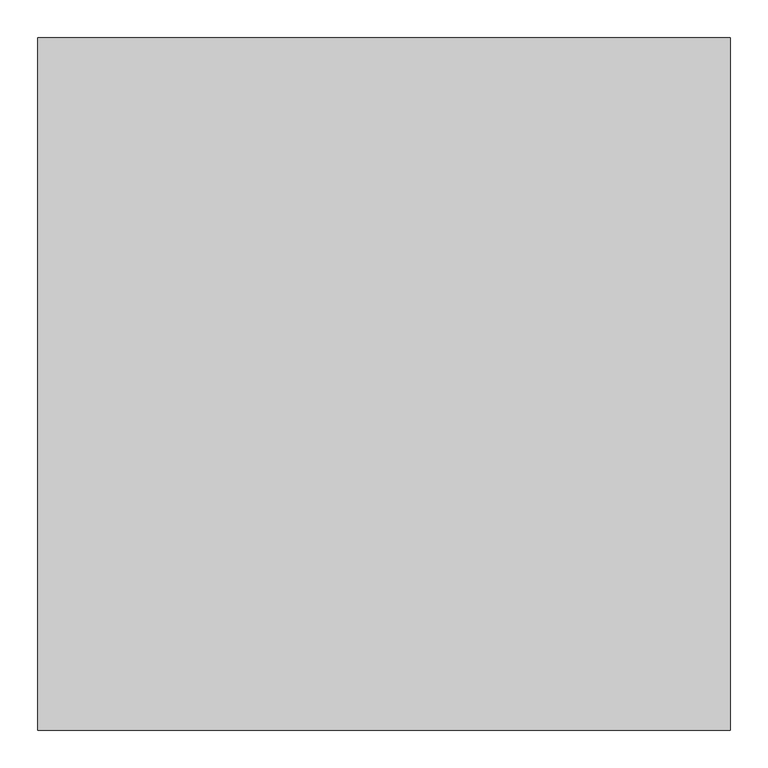
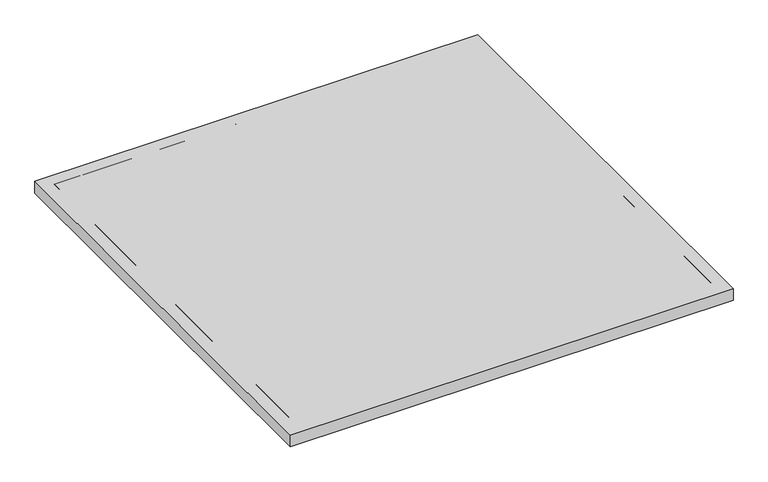
"""IFC4 building model written with IfcOpenShell, lengths in millimetres: proxy geometry, A6046 - Artwork, Decorative, With Frame : A6046 - Artwork, Decorative, With Frame."""

import ifcopenshell
import ifcopenshell.guid

model = None  # the IFC model being written
_history = None  # IfcOwnerHistory: only IFC2X3 demands one
_inside = {}  # id of a spatial element -> (the spatial element, [elements in it])
_under = {}  # id of a project, library or spatial element -> (it, [spatial elements below it])
_declared = {}  # id of a project -> (the project, [libraries it declares])
_typed = {}  # id of a type object -> (the type object, [elements of that type])
_made_of = {}  # id of a material, layer set ... -> (it, [elements and type objects made of it])


def new_model(schema):
    """Start an empty IFC model of exactly this schema.

    Asked for "IFC4X3", IfcOpenShell would pick the latest addendum, in which some entities
    have other attributes; the version numbers below select the first issue.
    IFC2X3 requires an IfcOwnerHistory on every rooted entity: one is made here for all.
    """
    global model, _history
    if schema == "IFC4X3":
        model = ifcopenshell.file(schema_version=(4, 3, 0, 0))
    else:
        model = ifcopenshell.file(schema=schema)
    _inside.clear()
    _under.clear()
    _declared.clear()
    _typed.clear()
    _made_of.clear()
    _history = None
    if model.schema == "IFC2X3":
        org = make("IfcOrganization", Name="unknown")
        user = make(
            "IfcPersonAndOrganization",
            ThePerson=make("IfcPerson", FamilyName="unknown"),
            TheOrganization=org,
        )
        app = make(
            "IfcApplication",
            ApplicationDeveloper=org,
            Version="unknown",
            ApplicationFullName="unknown",
            ApplicationIdentifier="unknown",
        )
        _history = make(
            "IfcOwnerHistory",
            OwningUser=user,
            OwningApplication=app,
            ChangeAction="ADDED",
            CreationDate=0,
        )
    return model


def make(cls, **values):
    """One entity of the class cls with the attributes given. An attribute that is None is left unset."""
    return model.create_entity(
        cls, **{name: value for name, value in values.items() if value is not None}
    )


def rooted(cls, **values):
    """An entity with a GlobalId (a new one), such as an element, a storey or a relation."""
    return make(cls, GlobalId=ifcopenshell.guid.new(), OwnerHistory=_history, **values)


def si_unit(unit_type, name, prefix=None):
    """IfcSIUnit, for example si_unit("LENGTHUNIT", "METRE", prefix="MILLI")."""
    return make("IfcSIUnit", UnitType=unit_type, Prefix=prefix, Name=name)


def assignment(units):
    """IfcUnitAssignment: the units of a project."""
    return None if units is None else make("IfcUnitAssignment", Units=units)


def point(xyz):
    """IfcCartesianPoint."""
    return None if xyz is None else make("IfcCartesianPoint", Coordinates=xyz)


def direction(xyz):
    """IfcDirection."""
    return None if xyz is None else make("IfcDirection", DirectionRatios=xyz)


def frame(location, z_axis=None, x_axis=None):
    """IfcAxis2Placement3D, a coordinate frame: its origin and axes. An axis left out is left unset."""
    return make(
        "IfcAxis2Placement3D",
        Location=point(location),
        Axis=direction(z_axis),
        RefDirection=direction(x_axis),
    )


def origin():
    """The frame at (0, 0, 0) with its axes left unset."""
    return frame((0.0, 0.0, 0.0))


def origin_with_axes():
    """The frame at (0, 0, 0) with the z axis (0, 0, 1) and the x axis (1, 0, 0) written out."""
    return frame((0.0, 0.0, 0.0), z_axis=(0.0, 0.0, 1.0), x_axis=(1.0, 0.0, 0.0))


def place(relative_to, where):
    """IfcLocalPlacement: puts the frame where relative to a parent placement (None: the world)."""
    return make(
        "IfcLocalPlacement", PlacementRelTo=relative_to, RelativePlacement=where
    )


def context(
    kind, dimensions, precision=None, world=None, true_north=None, identifier=None
):
    """IfcGeometricRepresentationContext, for example the 3D "Model" context."""
    return make(
        "IfcGeometricRepresentationContext",
        ContextIdentifier=identifier,
        ContextType=kind,
        CoordinateSpaceDimension=dimensions,
        Precision=precision,
        WorldCoordinateSystem=world,
        TrueNorth=true_north,
    )


def project(units=None, contexts=None):
    """IfcProject with its units and contexts."""
    return rooted(
        "IfcProject",
        Name="project",
        RepresentationContexts=contexts,
        UnitsInContext=assignment(units),
    )


def spatial(cls, under=None, at=None, **own):
    """A site, building, storey or space (cls), placed at a placement, below another one or the project."""
    s = rooted(cls, ObjectPlacement=at, **own)
    if under is not None:
        _under.setdefault(under.id(), (under, []))[1].append(s)
    return s


def polyline(points):
    """IfcPolyline through the points."""
    return make("IfcPolyline", Points=[point(p) for p in points])


def outline(outer, holes=None, kind="AREA"):
    """IfcArbitraryClosedProfileDef: a profile drawn as a closed curve; with holes, ...WithVoids."""
    if holes is None:
        return make("IfcArbitraryClosedProfileDef", ProfileType=kind, OuterCurve=outer)
    return make(
        "IfcArbitraryProfileDefWithVoids",
        ProfileType=kind,
        OuterCurve=outer,
        InnerCurves=holes,
    )


def extrude(swept, where, along, depth):
    """IfcExtrudedAreaSolid: the profile swept, set in the frame where, extruded along a direction by depth."""
    return make(
        "IfcExtrudedAreaSolid",
        SweptArea=swept,
        Position=where,
        ExtrudedDirection=direction(along),
        Depth=depth,
    )


def faces_of(points, faces, orient=None, outer=None):
    """IfcFace entities. A face is a list of loops; a loop is a list of indices into points, from 0.

    orient and outer hold one flag for each loop. By default every Orientation is true, the
    first loop of a face is its IfcFaceOuterBound and the others are IfcFaceBound.
    """
    made = []
    for i, loops in enumerate(faces):
        bounds = []
        for j, loop in enumerate(loops):
            is_outer = j == 0 if outer is None else outer[i][j]
            bounds.append(
                make(
                    "IfcFaceOuterBound" if is_outer else "IfcFaceBound",
                    Bound=make("IfcPolyLoop", Polygon=[points[k] for k in loop]),
                    Orientation=True if orient is None else orient[i][j],
                )
            )
        made.append(make("IfcFace", Bounds=bounds))
    return made


def faceted_brep(points, faces, orient=None, outer=None, voids=None):
    """IfcFacetedBrep: a solid bounded by flat faces; with voids (closed shells), ...WithVoids."""
    shared = [point(p) for p in points]
    hull = make("IfcClosedShell", CfsFaces=faces_of(shared, faces, orient, outer))
    if voids is None:
        return make("IfcFacetedBrep", Outer=hull)
    return make(
        "IfcFacetedBrepWithVoids",
        Outer=hull,
        Voids=[
            make(cls, CfsFaces=faces_of(shared, fs, o, b)) for cls, fs, o, b in voids
        ],
    )


def shape(context_of_items, identifier, shape_type, items):
    """IfcShapeRepresentation: the items that make up one representation, for example the "Body"."""
    return make(
        "IfcShapeRepresentation",
        ContextOfItems=context_of_items,
        RepresentationIdentifier=identifier,
        RepresentationType=shape_type,
        Items=items,
    )


def source(mapping_origin, context_of_items, identifier, shape_type, items):
    """IfcRepresentationMap: a shape defined once, which mapped items show again and again."""
    return make(
        "IfcRepresentationMap",
        MappingOrigin=mapping_origin,
        MappedRepresentation=shape(context_of_items, identifier, shape_type, items),
    )


def transform(
    local_origin,
    x_axis=None,
    y_axis=None,
    z_axis=None,
    scale=None,
    scale2=None,
    scale3=None,
    uniform=True,
):
    """IfcCartesianTransformationOperator3D, or its non-uniform kind. x_axis, y_axis, z_axis: its Axis1, 2, 3."""
    if uniform:
        return make(
            "IfcCartesianTransformationOperator3D",
            Axis1=direction(x_axis),
            Axis2=direction(y_axis),
            LocalOrigin=point(local_origin),
            Scale=scale,
            Axis3=direction(z_axis),
        )
    return make(
        "IfcCartesianTransformationOperator3DnonUniform",
        Axis1=direction(x_axis),
        Axis2=direction(y_axis),
        LocalOrigin=point(local_origin),
        Scale=scale,
        Axis3=direction(z_axis),
        Scale2=scale2,
        Scale3=scale3,
    )


def mapped(mapping_source, mapping_target):
    """IfcMappedItem: shows the shape of a source again, moved by a transform."""
    return make(
        "IfcMappedItem", MappingSource=mapping_source, MappingTarget=mapping_target
    )


def made_of(thing, what):
    """Note that an element or type object is made of a material, layer set ...; save() writes the relation."""
    if what is not None:
        _made_of.setdefault(what.id(), (what, []))[1].append(thing)
    return thing


def element(
    cls,
    number,
    at=None,
    inside=None,
    cuts=None,
    type_object=None,
    material=None,
    context=None,
    identifier="Body",
    shape_type=None,
    held_by="IfcProductDefinitionShape",
    body=None,
    shapes=None,
    **own,
):
    """One element of the class cls, such as IfcWall. Its Tag is "e" and its number.

    at: its placement. inside: the storey or other place that contains it. cuts: it is an
    opening in that element (IfcRelVoidsElement). A single representation is given by context,
    identifier, shape_type and body (its items); several are given by shapes. held_by: the class
    of the entity that holds the representations. save() writes the other relations.
    """
    e = rooted(cls, Tag="e%d" % number, ObjectPlacement=at, **own)
    if body is not None:
        shapes = [shape(context, identifier, shape_type, body)]
    if shapes is not None:
        e.Representation = make(held_by, Representations=shapes)
    if inside is not None:
        _inside.setdefault(inside.id(), (inside, []))[1].append(e)
    if cuts is not None:
        rooted(
            "IfcRelVoidsElement", RelatingBuildingElement=cuts, RelatedOpeningElement=e
        )
    if type_object is not None:
        _typed.setdefault(type_object.id(), (type_object, []))[1].append(e)
    return made_of(e, material)


def aggregate(whole, parts):
    """IfcRelAggregates: a whole, such as a stair, and the parts it consists of."""
    return rooted("IfcRelAggregates", RelatingObject=whole, RelatedObjects=parts)


def save(model, path):
    """Write the relations noted so far, then the file.

    IfcRelAggregates (storeys below a building ...), IfcRelContainedInSpatialStructure (elements
    in a storey), IfcRelDefinesByType, IfcRelAssociatesMaterial and IfcRelDeclares: one each for
    every whole, place, type object, material and project.
    """
    for whole, parts in _under.values():
        aggregate(whole, parts)
    for where, things in _inside.values():
        rooted(
            "IfcRelContainedInSpatialStructure",
            RelatedElements=things,
            RelatingStructure=where,
        )
    for kind, things in _typed.values():
        rooted("IfcRelDefinesByType", RelatedObjects=things, RelatingType=kind)
    for what, things in _made_of.values():
        rooted("IfcRelAssociatesMaterial", RelatedObjects=things, RelatingMaterial=what)
    for by, libraries in _declared.values():
        rooted("IfcRelDeclares", RelatingContext=by, RelatedDefinitions=libraries)
    model.write(path)


def specialty_equipment_89782f33(model_context):
    return source(origin(), model_context, "Body", "SolidModel", [
        extrude(outline(polyline([(457.2, 914.4), (457.2, 0.0), (-457.2, 0.0), (-457.2, 914.4), (457.2, 914.4)])), origin_with_axes(), (0.0, 0.0, 1.0), 25.4),
        extrude(outline(polyline([(431.8, 889.0), (431.8, 25.4), (-431.8, 25.4), (-431.8, 889.0), (431.8, 889.0)])), frame((0.0, 0.0, 12.7), z_axis=(0.0, 0.0, 1.0), x_axis=(1.0, 0.0, 0.0)), (0.0, 0.0, 1.0), 12.7),
        faceted_brep([(457.2, 914.4, 25.4), (457.2, 914.4, 0.0), (-457.2, 914.4, 0.0), (-457.2, 914.4, 25.4), (457.2, 0.0, 25.4), (-457.2, 0.0, 25.4), (-457.2, 0.0, 0.0), (457.2, 0.0, 0.0), (431.8, 889.0, 25.4), (431.8, 25.4, 25.4), (-431.8, 25.4, 25.4), (-431.8, 889.0, 25.4), (-431.8, 889.0, 12.7), (431.8, 889.0, 12.7), (431.8, 25.4, 12.7), (-431.8, 25.4, 12.7)], [[[0, 1, 2, 3]], [[4, 5, 6, 7]], [[3, 5, 4, 0], [8, 9, 10, 11]], [[2, 6, 5, 3]], [[1, 7, 6, 2]], [[0, 4, 7, 1]], [[8, 11, 12, 13]], [[10, 9, 14, 15]], [[11, 10, 15, 12]], [[12, 15, 14, 13]], [[13, 14, 9, 8]]]),
    ])


if __name__ == "__main__":
    model = new_model("IFC4")
    model_context = context("Model", 3, world=origin())
    ifc_project = project(units=[si_unit("LENGTHUNIT", "METRE", prefix="MILLI")], contexts=[model_context])
    site = spatial("IfcSite", under=ifc_project)
    building = spatial("IfcBuilding", under=site)
    placement = place(None, origin())
    specialty_equipment_shape = specialty_equipment_89782f33(model_context)
    element("IfcBuildingElementProxy", 1, Name="A6046 - Artwork, Decorative, With Frame : A6046 - Artwork, Decorative, With Frame", ObjectType="A6046 - Artwork, Decorative, With Frame : A6046 - Artwork, Decorative, With Frame", at=placement, inside=building, context=model_context, shape_type="MappedRepresentation", body=[
        mapped(specialty_equipment_shape, transform((0.0, 0.0, 0.0), x_axis=(1.0, 0.0, 0.0), y_axis=(0.0, 1.0, 0.0), z_axis=(0.0, 0.0, 1.0))),
    ])
    save(model, "model.ifc")

# Revit data of these elements
# Type "A6046 - Artwork, Decorative, With Frame : A6046 - Artwork, Decorative, With Frame"
#   Watts2 = "0"
#   Watts1 = "0"
#   Unit_Issue = "EA"
#   UTIL_6_Misc = "-"
#   UTIL_5_NonMedGas = "-"
#   UTIL_4_MiscGas = "-"
#   UTIL_3_MedGas = "-"
#   UTIL_2_Elec = "-"
#   UTIL_1_WaterDrain = "-"
#   Nomenclature = "Artwork, Decorative, With Frame"
#   NSN = "6230"
#   Location [instance default] = ""
#   JSN = "A6046"
#   Fund_Source_VA = "-"
#   Fund_Source_Navy = "-"
#   Fund_Source_Army = "-"
#   Fund_Source_AF = "-"
#   ELEC_Volts2 = "0"
#   ELEC_Volts1 = "0"
#   ELEC_Phase2 = "0"
#   ELEC_Phase1 = "0"
#   ELEC_HertzSwitch = "0"
#   ELEC_HertzDependent = "0"
#   ELEC_Hertz = "0"
#   ELEC_Amps2 = "0"
#   ELEC_Amps1 = "0"
#   DetailDescription = "This JSN is to be used for determining and defining location of decorative artwork."
#   CAT_VA = "C"
#   CAT_Navy = "C"
#   CAT_IHS = "-"
#   CAT_Army = "C"
#   CAT_AF = "C"
#   BTUperhour = "0"
#   Weight_IP = 0
#   Default Elevation = 7' - 0"
#   DIM_Width_IP = 0' - 0"
#   DIM_Height_IP = 0' - 0"
#   DIM_Depth_IP = 0' - 0"
#   CustomLength [instance default] = 3' - 0"
#   CustomHeight [instance default] = 3' - 0"
# Element 1 (IfcBuildingElementProxy, "A6046 - Artwork, Decorative, With Frame : A6046 - Artwork, Decorative, With Frame")
#   Location = "BRII2"
#   Materials on its faces: "Frame - Wood", "EquipSpace", "Picture"
# Materials
#   "Frame - Wood": class "Miscellaneous", colour RGB 66 39 32, transparency 0
#   "EquipSpace": class "Unassigned", colour RGB 221 217 195, transparency 0.5
#   "Picture": class "Miscellaneous", colour RGB 196 197 177, transparency 0
